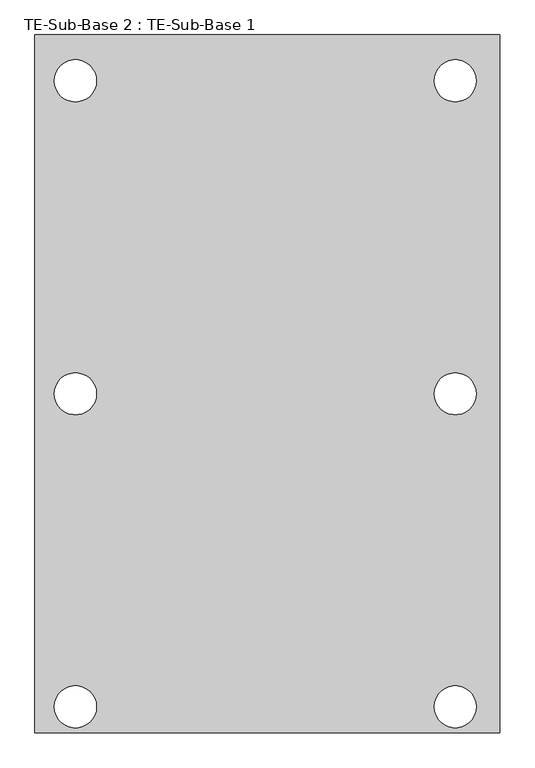
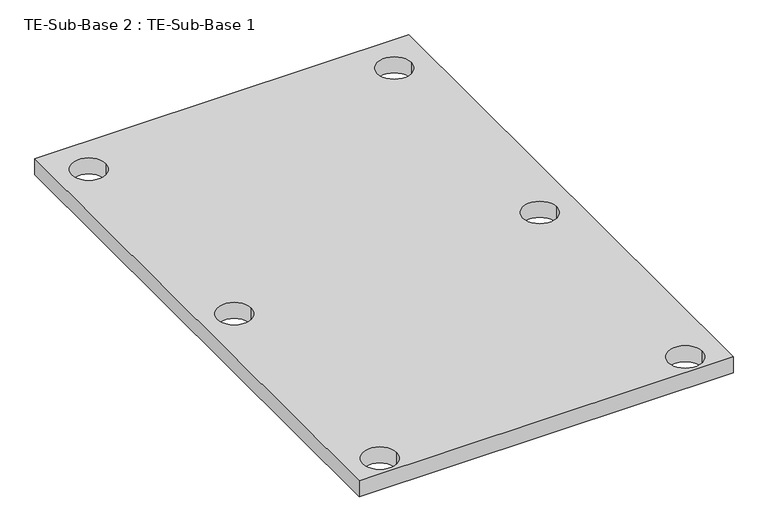
"""IFC4 building model written with IfcOpenShell, lengths in millimetres: proxy geometry, TE-Sub-Base 2 : TE-Sub-Base 1."""

from ifc_helpers import new_model, si_unit, point, frame, frame_2d, origin, place, context, project, spatial, polyline, circle_curve, trimmed, segment, composite_curve, outline, extrude, source, transform, mapped, element, save


def te_sub_base_2_te_sub_base_1_1fbd61a2(model_context):
    return source(origin(), model_context, "Body", "SweptSolid", [
        extrude(outline(polyline([(590544.8558739, -536503.3163358), (587173.7141748, -536503.3163358), (587173.7141748, -531442.3806716), (590544.8558739, -531442.3806716), (590544.8558739, -536503.3163358)]), holes=[composite_curve([segment(trimmed(circle_curve(frame_2d((587467.4934739, -531775.7413841)), 152.4), [point((587315.0934739, -531775.7413841))], [point((587619.8934739, -531775.7413841))], True, "CARTESIAN"), True, "CONTINUOUS"), segment(trimmed(circle_curve(frame_2d((587467.4934739, -531775.7413841)), 152.4), [point((587619.8934739, -531775.7413841))], [point((587315.0934739, -531775.7413841))], True, "CARTESIAN"), True, "CONTINUOUS")], self_intersect=False), composite_curve([segment(trimmed(circle_curve(frame_2d((590220.6835267, -531775.7413841)), 152.4), [point((590068.2835267, -531775.7413841))], [point((590373.0835267, -531775.7413841))], True, "CARTESIAN"), True, "CONTINUOUS"), segment(trimmed(circle_curve(frame_2d((590220.6835267, -531775.7413841)), 152.4), [point((590373.0835267, -531775.7413841))], [point((590068.2835267, -531775.7413841))], True, "CARTESIAN"), True, "CONTINUOUS")], self_intersect=False), composite_curve([segment(trimmed(circle_curve(frame_2d((590220.6835267, -534045.8663841)), 152.4), [point((590068.2835267, -534045.8663841))], [point((590373.0835267, -534045.8663841))], True, "CARTESIAN"), True, "CONTINUOUS"), segment(trimmed(circle_curve(frame_2d((590220.6835267, -534045.8663841)), 152.4), [point((590373.0835267, -534045.8663841))], [point((590068.2835267, -534045.8663841))], True, "CARTESIAN"), True, "CONTINUOUS")], self_intersect=False), composite_curve([segment(trimmed(circle_curve(frame_2d((587467.4934739, -534045.8663841)), 152.4), [point((587315.0934739, -534045.8663841))], [point((587619.8934739, -534045.8663841))], True, "CARTESIAN"), True, "CONTINUOUS"), segment(trimmed(circle_curve(frame_2d((587467.4934739, -534045.8663841)), 152.4), [point((587619.8934739, -534045.8663841))], [point((587315.0934739, -534045.8663841))], True, "CARTESIAN"), True, "CONTINUOUS")], self_intersect=False), composite_curve([segment(trimmed(circle_curve(frame_2d((587467.4934739, -536315.9913841)), 152.4), [point((587315.0934739, -536315.9913841))], [point((587619.8934739, -536315.9913841))], True, "CARTESIAN"), True, "CONTINUOUS"), segment(trimmed(circle_curve(frame_2d((587467.4934739, -536315.9913841)), 152.4), [point((587619.8934739, -536315.9913841))], [point((587315.0934739, -536315.9913841))], True, "CARTESIAN"), True, "CONTINUOUS")], self_intersect=False), composite_curve([segment(trimmed(circle_curve(frame_2d((590220.6835267, -536315.9913841)), 152.4), [point((590068.2835267, -536315.9913841))], [point((590373.0835267, -536315.9913841))], True, "CARTESIAN"), True, "CONTINUOUS"), segment(trimmed(circle_curve(frame_2d((590220.6835267, -536315.9913841)), 152.4), [point((590373.0835267, -536315.9913841))], [point((590068.2835267, -536315.9913841))], True, "CARTESIAN"), True, "CONTINUOUS")], self_intersect=False)]), frame((0.0, 0.0, -304.8), z_axis=(0.0, 0.0, 1.0), x_axis=(1.0, 0.0, 0.0)), (0.0, 0.0, 1.0), 152.4),
    ])


if __name__ == "__main__":
    model = new_model("IFC4")
    model_context = context("Model", 3, world=origin())
    ifc_project = project(units=[si_unit("LENGTHUNIT", "METRE", prefix="MILLI")], contexts=[model_context])
    site = spatial("IfcSite", under=ifc_project)
    building = spatial("IfcBuilding", under=site)
    placement = place(None, origin())
    te_sub_base_2_te_sub_base_1_shape = te_sub_base_2_te_sub_base_1_1fbd61a2(model_context)
    element("IfcBuildingElementProxy", 1, Name="TE-Sub-Base 2 : TE-Sub-Base 1", ObjectType="TE-Sub-Base 2 : TE-Sub-Base 1", at=placement, inside=building, context=model_context, shape_type="MappedRepresentation", body=[
        mapped(te_sub_base_2_te_sub_base_1_shape, transform((0.0, 0.0, 0.0), x_axis=(1.0, 0.0, 0.0), y_axis=(0.0, 1.0, 0.0), z_axis=(0.0, 0.0, 1.0))),
    ])
    save(model, "model.ifc")

# Revit data of these elements
# Element 1 (IfcBuildingElementProxy, "TE-Sub-Base 2 : TE-Sub-Base 1")
#   Materials on its faces: "#57 STONE COMPACTED TO 95% ASTM 1557"
# Materials
#   "#57 STONE COMPACTED TO 95% ASTM 1557": class "Generic", colour RGB 179 183 179, transparency 0, Cost = 0
